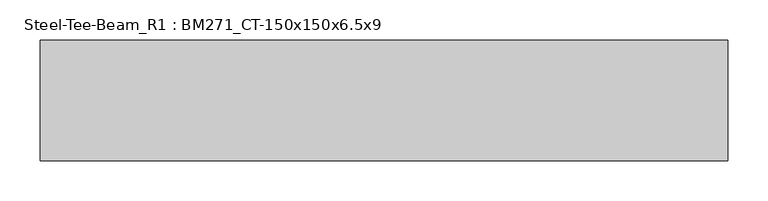
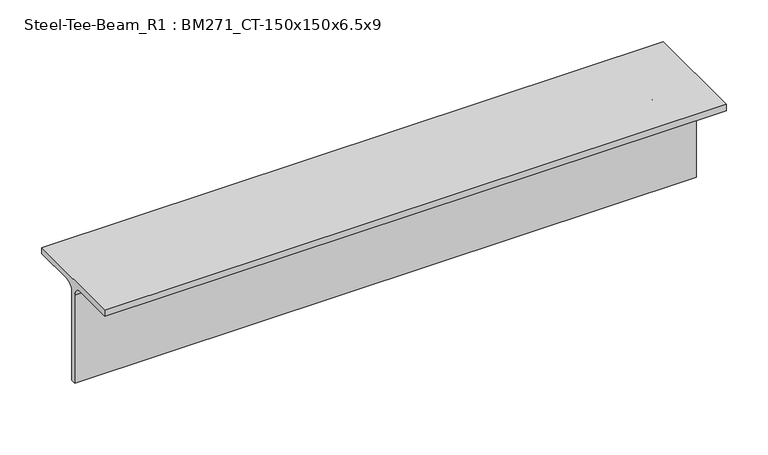
"""IFC4 building model written with IfcOpenShell, lengths in millimetres: member geometry, Steel-Tee-Beam_R1 : BM271_CT-150x150x6.5x9."""

from ifc_helpers import new_model, si_unit, point, frame, frame_2d, origin, place, context, project, spatial, polyline, circle_curve, trimmed, segment, composite_curve, outline, extrude, source, transform, mapped, element, save


def steel_tee_beam_r1_bm271_ct_150x150x6_5x9_4f0f3063(model_context):
    return source(origin(), model_context, "Body", "SweptSolid", [
        extrude(outline(composite_curve([segment(polyline([(75.0, 75.0), (75.0, 66.0), (16.25, 66.0)]), True, "CONTINUOUS"), segment(trimmed(circle_curve(frame_2d((16.25, 53.0)), 13.0), [point((16.25, 66.0))], [point((3.25, 53.0))], True, "CARTESIAN"), True, "CONTINUOUS"), segment(polyline([(3.25, 53.0), (3.25, -75.0), (-3.25, -75.0), (-3.25, 53.0)]), True, "CONTINUOUS"), segment(trimmed(circle_curve(frame_2d((-16.25, 53.0)), 13.0), [point((-3.25, 53.0))], [point((-16.25, 66.0))], True, "CARTESIAN"), True, "CONTINUOUS"), segment(polyline([(-16.25, 66.0), (-75.0, 66.0), (-75.0, 75.0), (75.0, 75.0)]), True, "CONTINUOUS")], self_intersect=False)), frame((-356.1687518, 0.0, 0.0), z_axis=(1.0, 0.0, 0.0), x_axis=(0.0, 1.0, 0.0)), (0.0, 0.0, 1.0), 856.1687518),
    ])


if __name__ == "__main__":
    model = new_model("IFC4")
    model_context = context("Model", 3, world=origin())
    ifc_project = project(units=[si_unit("LENGTHUNIT", "METRE", prefix="MILLI")], contexts=[model_context])
    site = spatial("IfcSite", under=ifc_project)
    building = spatial("IfcBuilding", under=site)
    placement = place(None, origin())
    steel_tee_beam_r1_bm271_ct_150x150x6_5x9_shape = steel_tee_beam_r1_bm271_ct_150x150x6_5x9_4f0f3063(model_context)
    element("IfcMember", 1, ObjectType="Steel-Tee-Beam_R1 : BM271_CT-150x150x6.5x9", at=placement, inside=building, context=model_context, shape_type="MappedRepresentation", body=[
        mapped(steel_tee_beam_r1_bm271_ct_150x150x6_5x9_shape, transform((0.0, 0.0, 0.0), x_axis=(1.0, 0.0, 0.0), y_axis=(0.0, 1.0, 0.0), z_axis=(0.0, 0.0, 1.0))),
    ])
    save(model, "model.ifc")

# Revit data of these elements
# Type "Steel-Tee-Beam_R1 : BM271_CT-150x150x6.5x9"
#   Keynote = "CT-150x150x6.5x9"
#   Surface Area = 0.588841 m²/m
#   Section Area = 23.3904 cm²
#   Mass per Unit Length = 18.3614 kg/m
#   Length [instance default] = 1.5240 m
#   bf = 0.1500 m
#   d = 0.1500 m
#   k = 0.0220 m
#   r = 0.0130 m
#   tf = 0.0090 m
#   tw = 0.0065 m
#   hec_material4 [instance default] = none
#   hec_material3 [instance default] = none
#   hec_material2 [instance default] = none
#   hec_material1 [instance default] = none
#   Structural Material [instance default] = Steel, 45-345
#   Assembly Code = ""
# Element 1 (IfcMember, "Steel-Tee-Beam_R1 : BM271_CT-150x150x6.5x9")
#   Structural Material = none
# Materials
#   "Steel, 45-345": class "Metal", colour RGB 189 187 185, transparency 0, Description = "Steel 345 MPa", Cost = 0
